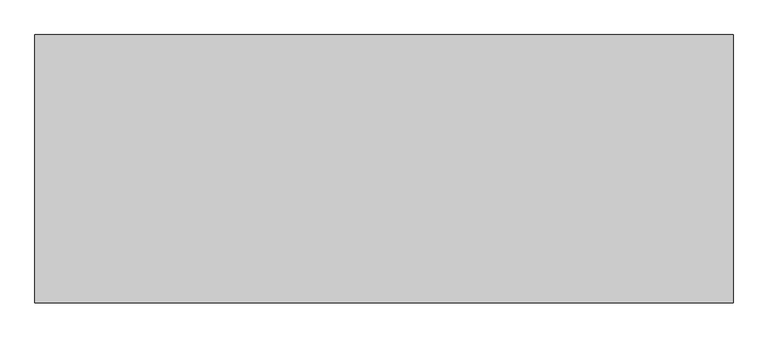
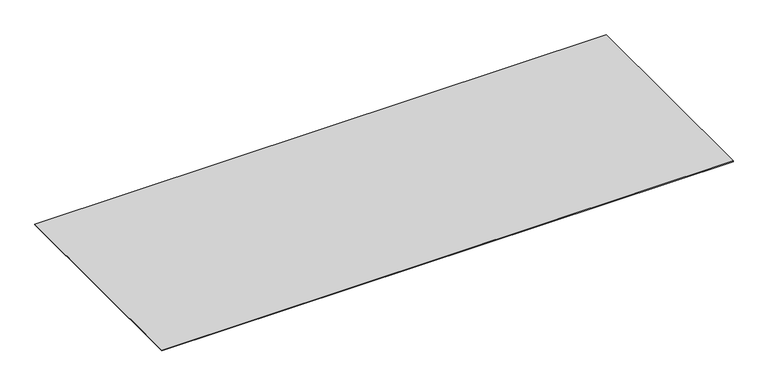
"""IFC4 building model written with IfcOpenShell, lengths in millimetres: proxy geometry, Generic Models 7:Generic Models 1:6:Generic Models 1:6 : Generic Models 7:Generic Models 1:337419:3 : Generic Models 7:Generic Models 1:6:Generic Models 1:6 : Generic Models 7:Generic Models 1:337419:312901."""

from ifc_helpers import new_model, si_unit, frame, origin, place, context, project, spatial, polyline, outline, extrude, source, transform, mapped, element, save


def generic_models_c0ab2777(model_context):
    return source(origin(), model_context, "Body", "SweptSolid", [
        extrude(outline(polyline([(667331.4117239, -536773.1913841), (667331.4117239, -578873.6913841), (557771.6867239, -578873.6913841), (557771.6867239, -536773.1913841), (667331.4117239, -536773.1913841)])), frame((0.0, 0.0, -158.1372439), z_axis=(0.0, 0.0, 1.0), x_axis=(1.0, 0.0, 0.0)), (0.0, 0.0, 1.0), 158.1372439),
    ])


if __name__ == "__main__":
    model = new_model("IFC4")
    model_context = context("Model", 3, world=origin())
    ifc_project = project(units=[si_unit("LENGTHUNIT", "METRE", prefix="MILLI")], contexts=[model_context])
    site = spatial("IfcSite", under=ifc_project)
    building = spatial("IfcBuilding", under=site)
    placement = place(None, origin())
    generic_models_shape = generic_models_c0ab2777(model_context)
    element("IfcBuildingElementProxy", 1, Name="Generic Models 7:Generic Models 1:6:Generic Models 1:6 : Generic Models 7:Generic Models 1:337419:3 : Generic Models 7:Generic Models 1:6:Generic Models 1:6 : Generic Models 7:Generic Models 1:337419:312901", ObjectType="Generic Models 7:Generic Models 1:6:Generic Models 1:6 : Generic Models 7:Generic Models 1:337419:3 : Generic Models 7:Generic Models 1:6:Generic Models 1:6 : Generic Models 7:Generic Models 1:337419:312901", at=placement, inside=building, context=model_context, shape_type="MappedRepresentation", body=[
        mapped(generic_models_shape, transform((0.0, 0.0, 0.0), x_axis=(1.0, 0.0, 0.0), y_axis=(0.0, 1.0, 0.0), z_axis=(0.0, 0.0, 1.0))),
    ])
    save(model, "model.ifc")

# Revit data of these elements
# Type "Generic Models 7:Generic Models 1:6:Generic Models 1:6 : Generic Models 7:Generic Models 1:337419:3 : Generic Models 7:Generic Models 1:6:Generic Models 1:6 : Generic Models 7:Generic Models 1:337419:312901"
#   NameOverride = "Generic Models 7:Generic Models 1:6:Generic Models 1:6 : Generic Models 7:Generic Models 1:337419:312901"
#   ObjectTypeOverride = "Generic Models 1:6 : Generic Models 7:Generic Models 1:337419"
#   Reference = "Generic Models 1"
#   Tag = "312901"
# Element 1 (IfcBuildingElementProxy, "Generic Models 7:Generic Models 1:6:Generic Models 1:6 : Generic Models 7:Generic Models 1:337419:3 : Generic Models 7:Generic Models 1:6:Generic Models 1:6 : Generic Models 7:Generic Models 1:337419:312901")
#   Materials on its faces: "CONCRETE SLAB - SEE STRUCT DWGS."
# Materials
#   "CONCRETE SLAB - SEE STRUCT DWGS.": class "Concrete", colour RGB 115 116 108, transparency 0, Description = "Lightweight concrete", Cost = 0
